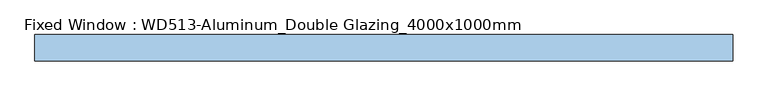
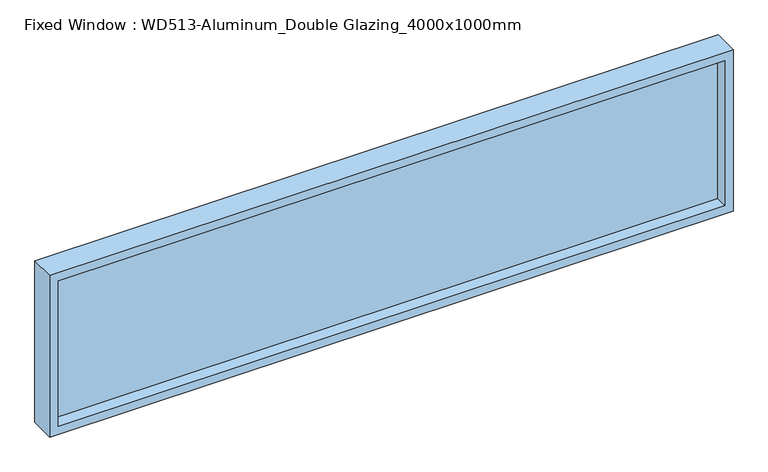
"""IFC4 building model written with IfcOpenShell, lengths in millimetres: window geometry, Fixed Window : WD513-Aluminum_Double Glazing_4000x1000mm."""

from ifc_helpers import new_model, si_unit, frame, origin, place, context, project, spatial, polyline, outline, extrude, source, transform, mapped, element, save


def fixed_window_wd513_aluminum_double_glazing_4000x1000mm_3ff382ba(model_context):
    return source(origin(), model_context, "Body", "SweptSolid", [
        extrude(outline(polyline([(-1950.0, 3.0), (1950.0, 3.0), (1950.0, -3.0), (-1950.0, -3.0), (-1950.0, 3.0)])), frame((0.0, 0.0, 850.0), z_axis=(0.0, 0.0, 1.0), x_axis=(1.0, 0.0, 0.0)), (0.0, 0.0, 1.0), 900.0),
        extrude(outline(polyline([(1800.0, -2000.0), (800.0, -2000.0), (800.0, 2000.0), (1800.0, 2000.0), (1800.0, -2000.0)]), holes=[polyline([(1750.0, -1950.0), (1750.0, 1950.0), (850.0, 1950.0), (850.0, -1950.0), (1750.0, -1950.0)])]), frame((0.0, -75.0, 0.0), z_axis=(0.0, 1.0, 0.0), x_axis=(0.0, 0.0, 1.0)), (0.0, 0.0, 1.0), 150.0),
    ])


if __name__ == "__main__":
    model = new_model("IFC4")
    model_context = context("Model", 3, world=origin())
    ifc_project = project(units=[si_unit("LENGTHUNIT", "METRE", prefix="MILLI")], contexts=[model_context])
    site = spatial("IfcSite", under=ifc_project)
    building = spatial("IfcBuilding", under=site)
    placement = place(None, origin())
    fixed_window_wd513_aluminum_double_glazing_4000x1000mm_shape = fixed_window_wd513_aluminum_double_glazing_4000x1000mm_3ff382ba(model_context)
    element("IfcWindow", 1, ObjectType="Fixed Window : WD513-Aluminum_Double Glazing_4000x1000mm", at=placement, inside=building, context=model_context, shape_type="MappedRepresentation", body=[
        mapped(fixed_window_wd513_aluminum_double_glazing_4000x1000mm_shape, transform((0.0, 0.0, 0.0), x_axis=(1.0, 0.0, 0.0), y_axis=(0.0, 1.0, 0.0), z_axis=(0.0, 0.0, 1.0))),
    ])
    save(model, "model.ifc")

# Revit data of these elements
# Type "Fixed Window : WD513-Aluminum_Double Glazing_4000x1000mm"
#   Type Mark = "AW"
#   Analytic Construction = "<None>"
#   창 두께 = 0.1500 m
#   Height = 1.0000 m
#   절반 창 두께 = 0.0750 m
#   기본 씰 높이 = 0.8000 m
#   Width = 4.0000 m
#   Wall Closure = 3
#   Define Thermal Properties by = 1
#   창 패널 = AW2 창 패널
#   창 프레임 = A04AQ127-00002_Aluminum Window_None FP
#   Description = (empty or 0)
# Element 1 (IfcWindow, "Fixed Window : WD513-Aluminum_Double Glazing_4000x1000mm")
#   Materials on its faces: "A04AQ127-00002_Aluminum Window_None FP", "AW2 창 패널"
# Materials
#   "AW2 창 패널": class "유리", colour RGB 0 0 255, transparency 0.75
#   "A04AQ127-00002_Aluminum Window_None FP": class "금속", colour RGB 247 247 247, transparency 0, Cost = 0
